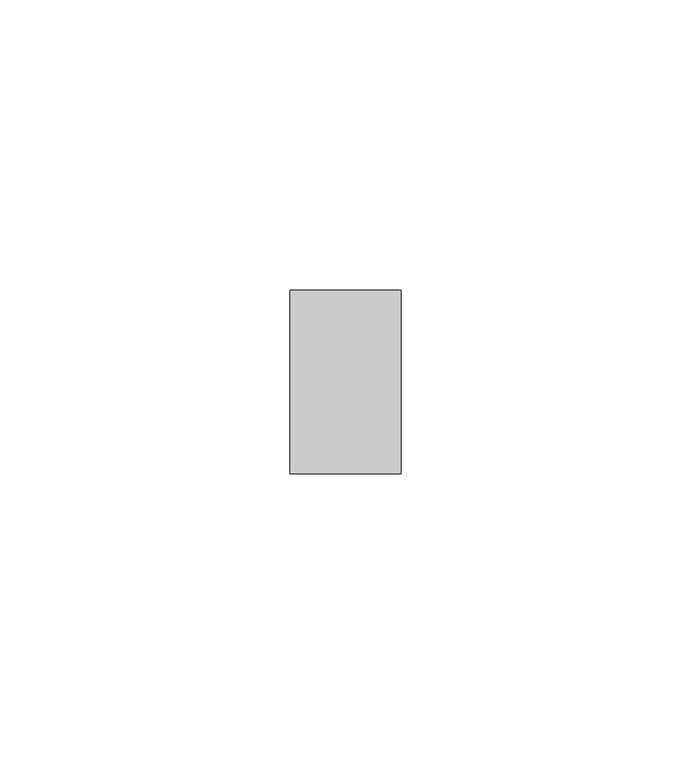
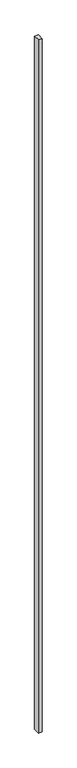
"""IFC4 building model written with IfcOpenShell, lengths in millimetres: proxy geometry, Generic Models 11:Generic Models 1:306267:Generic Models 1:306267 : Generic Models 11:Generic Models 1:306267:300405:Generic Models 1:306267:Generic Models 1:306267 : Generic Models 11:Generic Models 1:306267:300405 : Generic Models 11:Generic Models 1:306267:Generic Models 1:306267 : Generic Models 11:Generic Models 1:306267:300405:7 : Generic Models 11:Generic Models 1:306267:Generic Models 1:306267 : Generic Models 11:Generic Models 1:306267:300405:Generic Models 1:306267:Generic Models 1:306267 : Generic Models 11:Generic Models 1:306267:300405 : Generic Models 11:Generic Models 1:306267:Generic Models 1:306267 : Generic Models 11:Generic Models 1:306267:300405:300182."""

from ifc_helpers import new_model, si_unit, origin, origin_with_axes, place, context, project, spatial, polyline, outline, extrude, source, transform, mapped, element, save


def generic_models_0cc168be(model_context):
    return source(origin(), model_context, "Body", "SweptSolid", [
        extrude(outline(polyline([(569492.4356601, -579045.8399212), (569492.4356601, -579077.4247924), (569473.3856601, -579077.4247924), (569473.3856601, -579045.8399212), (569492.4356601, -579045.8399212)])), origin_with_axes(), (0.0, 0.0, 1.0), 3689.35),
    ])


if __name__ == "__main__":
    model = new_model("IFC4")
    model_context = context("Model", 3, world=origin())
    ifc_project = project(units=[si_unit("LENGTHUNIT", "METRE", prefix="MILLI")], contexts=[model_context])
    site = spatial("IfcSite", under=ifc_project)
    building = spatial("IfcBuilding", under=site)
    placement = place(None, origin())
    generic_models_shape = generic_models_0cc168be(model_context)
    element("IfcBuildingElementProxy", 1, Name="Generic Models 11:Generic Models 1:306267:Generic Models 1:306267 : Generic Models 11:Generic Models 1:306267:300405:Generic Models 1:306267:Generic Models 1:306267 : Generic Models 11:Generic Models 1:306267:300405 : Generic Models 11:Generic Models 1:306267:Generic Models 1:306267 : Generic Models 11:Generic Models 1:306267:300405:7 : Generic Models 11:Generic Models 1:306267:Generic Models 1:306267 : Generic Models 11:Generic Models 1:306267:300405:Generic Models 1:306267:Generic Models 1:306267 : Generic Models 11:Generic Models 1:306267:300405 : Generic Models 11:Generic Models 1:306267:Generic Models 1:306267 : Generic Models 11:Generic Models 1:306267:300405:300182", ObjectType="Generic Models 11:Generic Models 1:306267:Generic Models 1:306267 : Generic Models 11:Generic Models 1:306267:300405:Generic Models 1:306267:Generic Models 1:306267 : Generic Models 11:Generic Models 1:306267:300405 : Generic Models 11:Generic Models 1:306267:Generic Models 1:306267 : Generic Models 11:Generic Models 1:306267:300405:7 : Generic Models 11:Generic Models 1:306267:Generic Models 1:306267 : Generic Models 11:Generic Models 1:306267:300405:Generic Models 1:306267:Generic Models 1:306267 : Generic Models 11:Generic Models 1:306267:300405 : Generic Models 11:Generic Models 1:306267:Generic Models 1:306267 : Generic Models 11:Generic Models 1:306267:300405:300182", at=placement, inside=building, context=model_context, shape_type="MappedRepresentation", body=[
        mapped(generic_models_shape, transform((0.0, 0.0, 0.0), x_axis=(1.0, 0.0, 0.0), y_axis=(0.0, 1.0, 0.0), z_axis=(0.0, 0.0, 1.0))),
    ])
    save(model, "model.ifc")

# Revit data of these elements
# Type "Generic Models 11:Generic Models 1:306267:Generic Models 1:306267 : Generic Models 11:Generic Models 1:306267:300405:Generic Models 1:306267:Generic Models 1:306267 : Generic Models 11:Generic Models 1:306267:300405 : Generic Models 11:Generic Models 1:306267:Generic Models 1:306267 : Generic Models 11:Generic Models 1:306267:300405:7 : Generic Models 11:Generic Models 1:306267:Generic Models 1:306267 : Generic Models 11:Generic Models 1:306267:300405:Generic Models 1:306267:Generic Models 1:306267 : Generic Models 11:Generic Models 1:306267:300405 : Generic Models 11:Generic Models 1:306267:Generic Models 1:306267 : Generic Models 11:Generic Models 1:306267:300405:300182"
#   NameOverride = "Generic Models 11:Generic Models 1:306267:Generic Models 1:306267 : Generic Models 11:Generic Models 1:306267:300405:Generic Models 1:306267:Generic Models 1:306267 : Generic Models 11:Generic Models 1:306267:300405 : Generic Models 11:Generic Models 1:306267:Generic Models 1:306267 : Generic Models 11:Generic Models 1:306267:300405:300182"
#   ObjectTypeOverride = "Generic Models 1:306267:Generic Models 1:306267 : Generic Models 11:Generic Models 1:306267:300405 : Generic Models 11:Generic Models 1:306267:Generic Models 1:306267 : Generic Models 11:Generic Models 1:306267:300405"
#   Reference = "Generic Models 1"
#   Tag = "300182"
